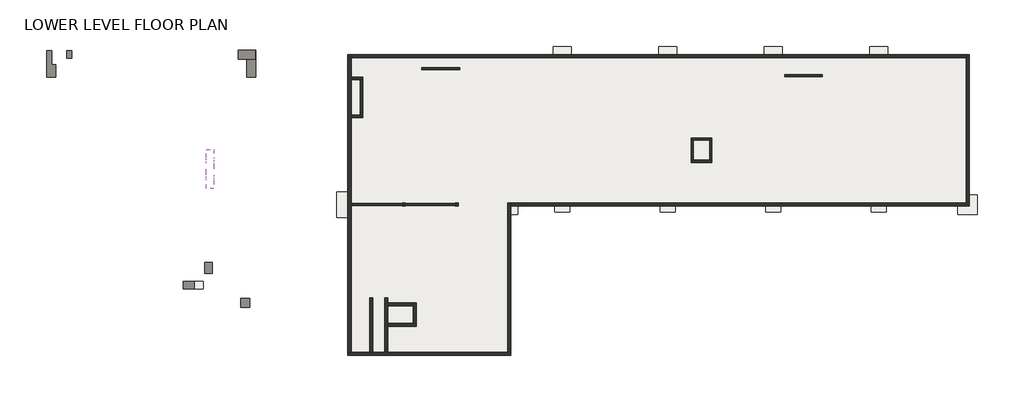
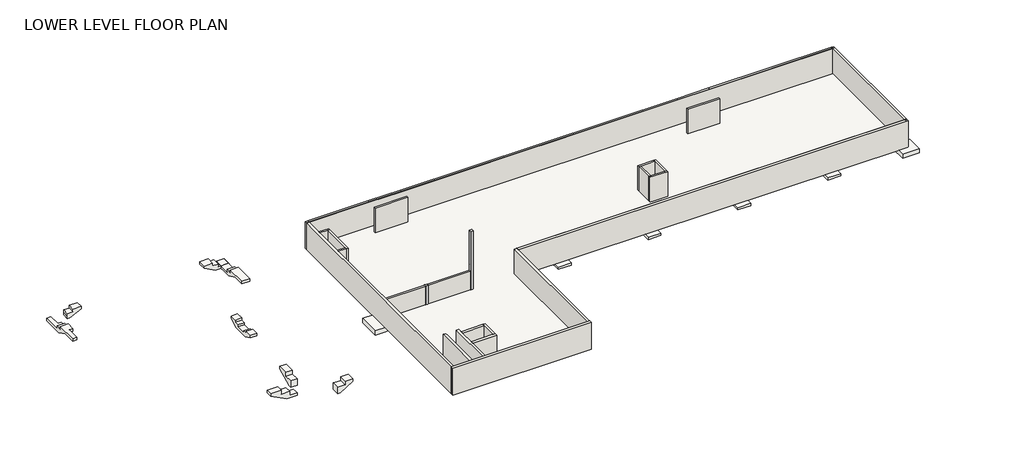
# One storey: 22 slabs, 22 walls, 2 columns.
"""IFC4 building model written with IfcOpenShell, lengths in millimetres."""

import ifcopenshell
import ifcopenshell.guid

model = None  # the IFC model being written
_history = None  # IfcOwnerHistory: only IFC2X3 demands one
_inside = {}  # id of a spatial element -> (the spatial element, [elements in it])
_under = {}  # id of a project, library or spatial element -> (it, [spatial elements below it])
_declared = {}  # id of a project -> (the project, [libraries it declares])
_typed = {}  # id of a type object -> (the type object, [elements of that type])
_made_of = {}  # id of a material, layer set ... -> (it, [elements and type objects made of it])


def new_model(schema):
    """Start an empty IFC model of exactly this schema.

    Asked for "IFC4X3", IfcOpenShell would pick the latest addendum, in which some entities
    have other attributes; the version numbers below select the first issue.
    IFC2X3 requires an IfcOwnerHistory on every rooted entity: one is made here for all.
    """
    global model, _history
    if schema == "IFC4X3":
        model = ifcopenshell.file(schema_version=(4, 3, 0, 0))
    else:
        model = ifcopenshell.file(schema=schema)
    _inside.clear()
    _under.clear()
    _declared.clear()
    _typed.clear()
    _made_of.clear()
    _history = None
    if model.schema == "IFC2X3":
        org = make("IfcOrganization", Name="unknown")
        user = make(
            "IfcPersonAndOrganization",
            ThePerson=make("IfcPerson", FamilyName="unknown"),
            TheOrganization=org,
        )
        app = make(
            "IfcApplication",
            ApplicationDeveloper=org,
            Version="unknown",
            ApplicationFullName="unknown",
            ApplicationIdentifier="unknown",
        )
        _history = make(
            "IfcOwnerHistory",
            OwningUser=user,
            OwningApplication=app,
            ChangeAction="ADDED",
            CreationDate=0,
        )
    return model


def make(cls, **values):
    """One entity of the class cls with the attributes given. An attribute that is None is left unset."""
    return model.create_entity(
        cls, **{name: value for name, value in values.items() if value is not None}
    )


def rooted(cls, **values):
    """An entity with a GlobalId (a new one), such as an element, a storey or a relation."""
    return make(cls, GlobalId=ifcopenshell.guid.new(), OwnerHistory=_history, **values)


def si_unit(unit_type, name, prefix=None):
    """IfcSIUnit, for example si_unit("LENGTHUNIT", "METRE", prefix="MILLI")."""
    return make("IfcSIUnit", UnitType=unit_type, Prefix=prefix, Name=name)


def assignment(units):
    """IfcUnitAssignment: the units of a project."""
    return None if units is None else make("IfcUnitAssignment", Units=units)


def point(xyz):
    """IfcCartesianPoint."""
    return None if xyz is None else make("IfcCartesianPoint", Coordinates=xyz)


def direction(xyz):
    """IfcDirection."""
    return None if xyz is None else make("IfcDirection", DirectionRatios=xyz)


def frame(location, z_axis=None, x_axis=None):
    """IfcAxis2Placement3D, a coordinate frame: its origin and axes. An axis left out is left unset."""
    return make(
        "IfcAxis2Placement3D",
        Location=point(location),
        Axis=direction(z_axis),
        RefDirection=direction(x_axis),
    )


def origin():
    """The frame at (0, 0, 0) with its axes left unset."""
    return frame((0.0, 0.0, 0.0))


def place(relative_to, where):
    """IfcLocalPlacement: puts the frame where relative to a parent placement (None: the world)."""
    return make(
        "IfcLocalPlacement", PlacementRelTo=relative_to, RelativePlacement=where
    )


def context(
    kind, dimensions, precision=None, world=None, true_north=None, identifier=None
):
    """IfcGeometricRepresentationContext, for example the 3D "Model" context."""
    return make(
        "IfcGeometricRepresentationContext",
        ContextIdentifier=identifier,
        ContextType=kind,
        CoordinateSpaceDimension=dimensions,
        Precision=precision,
        WorldCoordinateSystem=world,
        TrueNorth=true_north,
    )


def project(units=None, contexts=None):
    """IfcProject with its units and contexts."""
    return rooted(
        "IfcProject",
        Name="project",
        RepresentationContexts=contexts,
        UnitsInContext=assignment(units),
    )


def spatial(cls, under=None, at=None, **own):
    """A site, building, storey or space (cls), placed at a placement, below another one or the project."""
    s = rooted(cls, ObjectPlacement=at, **own)
    if under is not None:
        _under.setdefault(under.id(), (under, []))[1].append(s)
    return s


def polyline(points):
    """IfcPolyline through the points."""
    return make("IfcPolyline", Points=[point(p) for p in points])


def outline(outer, holes=None, kind="AREA"):
    """IfcArbitraryClosedProfileDef: a profile drawn as a closed curve; with holes, ...WithVoids."""
    if holes is None:
        return make("IfcArbitraryClosedProfileDef", ProfileType=kind, OuterCurve=outer)
    return make(
        "IfcArbitraryProfileDefWithVoids",
        ProfileType=kind,
        OuterCurve=outer,
        InnerCurves=holes,
    )


def extrude(swept, where, along, depth):
    """IfcExtrudedAreaSolid: the profile swept, set in the frame where, extruded along a direction by depth."""
    return make(
        "IfcExtrudedAreaSolid",
        SweptArea=swept,
        Position=where,
        ExtrudedDirection=direction(along),
        Depth=depth,
    )


def faces_of(points, faces, orient=None, outer=None):
    """IfcFace entities. A face is a list of loops; a loop is a list of indices into points, from 0.

    orient and outer hold one flag for each loop. By default every Orientation is true, the
    first loop of a face is its IfcFaceOuterBound and the others are IfcFaceBound.
    """
    made = []
    for i, loops in enumerate(faces):
        bounds = []
        for j, loop in enumerate(loops):
            is_outer = j == 0 if outer is None else outer[i][j]
            bounds.append(
                make(
                    "IfcFaceOuterBound" if is_outer else "IfcFaceBound",
                    Bound=make("IfcPolyLoop", Polygon=[points[k] for k in loop]),
                    Orientation=True if orient is None else orient[i][j],
                )
            )
        made.append(make("IfcFace", Bounds=bounds))
    return made


def faceted_brep(points, faces, orient=None, outer=None, voids=None):
    """IfcFacetedBrep: a solid bounded by flat faces; with voids (closed shells), ...WithVoids."""
    shared = [point(p) for p in points]
    hull = make("IfcClosedShell", CfsFaces=faces_of(shared, faces, orient, outer))
    if voids is None:
        return make("IfcFacetedBrep", Outer=hull)
    return make(
        "IfcFacetedBrepWithVoids",
        Outer=hull,
        Voids=[
            make(cls, CfsFaces=faces_of(shared, fs, o, b)) for cls, fs, o, b in voids
        ],
    )


def shape(context_of_items, identifier, shape_type, items):
    """IfcShapeRepresentation: the items that make up one representation, for example the "Body"."""
    return make(
        "IfcShapeRepresentation",
        ContextOfItems=context_of_items,
        RepresentationIdentifier=identifier,
        RepresentationType=shape_type,
        Items=items,
    )


def source(mapping_origin, context_of_items, identifier, shape_type, items):
    """IfcRepresentationMap: a shape defined once, which mapped items show again and again."""
    return make(
        "IfcRepresentationMap",
        MappingOrigin=mapping_origin,
        MappedRepresentation=shape(context_of_items, identifier, shape_type, items),
    )


def transform(
    local_origin,
    x_axis=None,
    y_axis=None,
    z_axis=None,
    scale=None,
    scale2=None,
    scale3=None,
    uniform=True,
):
    """IfcCartesianTransformationOperator3D, or its non-uniform kind. x_axis, y_axis, z_axis: its Axis1, 2, 3."""
    if uniform:
        return make(
            "IfcCartesianTransformationOperator3D",
            Axis1=direction(x_axis),
            Axis2=direction(y_axis),
            LocalOrigin=point(local_origin),
            Scale=scale,
            Axis3=direction(z_axis),
        )
    return make(
        "IfcCartesianTransformationOperator3DnonUniform",
        Axis1=direction(x_axis),
        Axis2=direction(y_axis),
        LocalOrigin=point(local_origin),
        Scale=scale,
        Axis3=direction(z_axis),
        Scale2=scale2,
        Scale3=scale3,
    )


def mapped(mapping_source, mapping_target):
    """IfcMappedItem: shows the shape of a source again, moved by a transform."""
    return make(
        "IfcMappedItem", MappingSource=mapping_source, MappingTarget=mapping_target
    )


def made_of(thing, what):
    """Note that an element or type object is made of a material, layer set ...; save() writes the relation."""
    if what is not None:
        _made_of.setdefault(what.id(), (what, []))[1].append(thing)
    return thing


def element(
    cls,
    number,
    at=None,
    inside=None,
    cuts=None,
    type_object=None,
    material=None,
    context=None,
    identifier="Body",
    shape_type=None,
    held_by="IfcProductDefinitionShape",
    body=None,
    shapes=None,
    **own,
):
    """One element of the class cls, such as IfcWall. Its Tag is "e" and its number.

    at: its placement. inside: the storey or other place that contains it. cuts: it is an
    opening in that element (IfcRelVoidsElement). A single representation is given by context,
    identifier, shape_type and body (its items); several are given by shapes. held_by: the class
    of the entity that holds the representations. save() writes the other relations.
    """
    e = rooted(cls, Tag="e%d" % number, ObjectPlacement=at, **own)
    if body is not None:
        shapes = [shape(context, identifier, shape_type, body)]
    if shapes is not None:
        e.Representation = make(held_by, Representations=shapes)
    if inside is not None:
        _inside.setdefault(inside.id(), (inside, []))[1].append(e)
    if cuts is not None:
        rooted(
            "IfcRelVoidsElement", RelatingBuildingElement=cuts, RelatedOpeningElement=e
        )
    if type_object is not None:
        _typed.setdefault(type_object.id(), (type_object, []))[1].append(e)
    return made_of(e, material)


def aggregate(whole, parts):
    """IfcRelAggregates: a whole, such as a stair, and the parts it consists of."""
    return rooted("IfcRelAggregates", RelatingObject=whole, RelatedObjects=parts)


def save(model, path):
    """Write the relations noted so far, then the file.

    IfcRelAggregates (storeys below a building ...), IfcRelContainedInSpatialStructure (elements
    in a storey), IfcRelDefinesByType, IfcRelAssociatesMaterial and IfcRelDeclares: one each for
    every whole, place, type object, material and project.
    """
    for whole, parts in _under.values():
        aggregate(whole, parts)
    for where, things in _inside.values():
        rooted(
            "IfcRelContainedInSpatialStructure",
            RelatedElements=things,
            RelatingStructure=where,
        )
    for kind, things in _typed.values():
        rooted("IfcRelDefinesByType", RelatedObjects=things, RelatingType=kind)
    for what, things in _made_of.values():
        rooted("IfcRelAssociatesMaterial", RelatedObjects=things, RelatingMaterial=what)
    for by, libraries in _declared.values():
        rooted("IfcRelDeclares", RelatingContext=by, RelatedDefinitions=libraries)
    model.write(path)


def footing_rectangular_4c268a4d(model_context):
    return source(origin(), model_context, "Body", "SweptSolid", [
        extrude(outline(polyline([(1295.4, 1295.4), (1295.4, -1295.4), (-1295.4, -1295.4), (-1295.4, 1295.4), (1295.4, 1295.4)])), frame((0.0, 0.0, -609.6), z_axis=(0.0, 0.0, 1.0), x_axis=(1.0, 0.0, 0.0)), (0.0, 0.0, 1.0), 609.6),
    ])


def footing_rectangular_a4ec12e7(model_context):
    return source(origin(), model_context, "Body", "SweptSolid", [
        extrude(outline(polyline([(1828.8, 1828.8), (1828.8, -1828.8), (-1828.8, -1828.8), (-1828.8, 1828.8), (1828.8, 1828.8)])), frame((0.0, 0.0, -609.6), z_axis=(0.0, 0.0, 1.0), x_axis=(1.0, 0.0, 0.0)), (0.0, 0.0, 1.0), 609.6),
    ])


def footing_rectangular_876cc71e(model_context):
    return source(origin(), model_context, "Body", "SweptSolid", [
        extrude(outline(polyline([(990.6, 990.6), (990.6, -990.6), (-990.6, -990.6), (-990.6, 990.6), (990.6, 990.6)])), frame((0.0, 0.0, -457.2), z_axis=(0.0, 0.0, 1.0), x_axis=(1.0, 0.0, 0.0)), (0.0, 0.0, 1.0), 457.2),
    ])


def footing_rectangular_0e916acc(model_context):
    return source(origin(), model_context, "Body", "SweptSolid", [
        extrude(outline(polyline([(1295.4, 1295.4), (1295.4, -1295.4), (-1295.4, -1295.4), (-1295.4, 1295.4), (1295.4, 1295.4)])), frame((0.0, 0.0, -508.0), z_axis=(0.0, 0.0, 1.0), x_axis=(1.0, 0.0, 0.0)), (0.0, 0.0, 1.0), 508.0),
    ])


def footing_rectangular_f5_f52d0094(model_context):
    return source(origin(), model_context, "Body", "SweptSolid", [
        extrude(outline(polyline([(762.0, 762.0), (762.0, -762.0), (-762.0, -762.0), (-762.0, 762.0), (762.0, 762.0)])), frame((0.0, 0.0, -304.8), z_axis=(0.0, 0.0, 1.0), x_axis=(1.0, 0.0, 0.0)), (0.0, 0.0, 1.0), 304.8),
    ])


def footing_rectangular_f6_e8c3e57f(model_context):
    return source(origin(), model_context, "Body", "SweptSolid", [
        extrude(outline(polyline([(914.4, 914.4), (914.4, -914.4), (-914.4, -914.4), (-914.4, 914.4), (914.4, 914.4)])), frame((0.0, 0.0, -304.8), z_axis=(0.0, 0.0, 1.0), x_axis=(1.0, 0.0, 0.0)), (0.0, 0.0, 1.0), 304.8),
    ])


def foundation_step_foundation_step_6eb52276(model_context):
    return source(origin(), model_context, "Body", "Brep", [
        faceted_brep([(-65781.2850821, 11238.2505048, -1422.4), (-65781.2850821, 11238.2505048, -1752.6), (-65781.2850821, 13409.3518471, -1752.6), (-65781.2850821, 13409.3518471, -2057.4), (-65781.2850821, 10933.4505048, -2057.4), (-65781.2850821, 9612.6505048, -1397.0), (-65781.2850821, 8050.5505048, -1397.0), (-65781.2850821, 8050.5505048, -1092.2), (-65781.2850821, 10577.8505048, -1092.2), (-65781.2850821, 10577.8505048, -1422.4), (-64866.8850821, 11238.2505048, -1752.6), (-64866.8850821, 11238.2505048, -1422.4), (-64866.8850821, 10577.8505048, -1422.4), (-64866.8850821, 10577.8505048, -1092.2), (-64866.8850821, 9574.5505048, -1092.2), (-64866.8850821, 9574.5505048, -1397.0), (-64866.8850821, 9612.6505048, -1397.0), (-64866.8850821, 10933.4505048, -2057.4), (-64866.8850821, 12012.9505048, -2057.4), (-64866.8850821, 12012.9505048, -1752.6), (-65273.2850821, 12012.9505048, -1752.6), (-65273.2850821, 13409.3518471, -1752.6), (-65273.2850821, 13409.3518471, -2057.4), (-65273.2850821, 12012.9505048, -2057.4), (-65273.2850821, 9574.5505048, -1397.0), (-65273.2850821, 8050.5505048, -1397.0), (-65273.2850821, 8050.5505048, -1092.2), (-65273.2850821, 9574.5505048, -1092.2)], [[[0, 1, 2, 3, 4, 5, 6, 7, 8, 9]], [[10, 11, 12, 13, 14, 15, 16, 17, 18, 19]], [[1, 0, 11, 10]], [[2, 1, 10, 19, 20, 21]], [[3, 2, 21, 22]], [[4, 3, 22, 23, 18, 17]], [[6, 5, 16, 15, 24, 25]], [[7, 6, 25, 26]], [[8, 7, 26, 27, 14, 13]], [[9, 8, 13, 12]], [[0, 9, 12, 11]], [[5, 4, 17, 16]], [[27, 24, 15, 14]], [[24, 27, 26, 25]], [[20, 23, 22, 21]], [[23, 20, 19, 18]]]),
    ])


def foundation_step1_foundation_step_c4984ecd(model_context):
    return source(origin(), model_context, "Body", "SweptSolid", [
        extrude(outline(polyline([(-1397.0, -62011.044558), (-1092.2, -62011.044558), (-1092.2, -62976.244558), (-1422.4, -62976.244558), (-1422.4, -63636.644558), (-1752.6, -63636.644558), (-1752.6, -63634.9850821), (-2057.4, -63634.9850821), (-2057.4, -63331.844558), (-1397.0, -62011.044558)])), frame((0.0, 12612.4268471, 0.0), z_axis=(0.0, 1.0, 0.0), x_axis=(0.0, 0.0, 1.0)), (0.0, 0.0, 1.0), 762.0),
    ])


def foundation_step2_foundation_step_839b83da(model_context):
    return source(origin(), model_context, "Body", "SweptSolid", [
        extrude(outline(polyline([(-1092.2, -46445.5350821), (-1092.2, -47410.7350821), (-1397.0, -47410.7350821), (-2057.4, -46089.9350821), (-2057.4, -44565.9350821), (-1752.6, -44565.9350821), (-1752.6, -45785.1350821), (-1422.4, -45785.1350821), (-1422.4, -46445.5350821), (-1092.2, -46445.5350821)])), frame((0.0, 12628.3018471, 0.0), z_axis=(0.0, 1.0, 0.0), x_axis=(0.0, 0.0, 1.0)), (0.0, 0.0, 1.0), 914.4),
    ])


def foundation_step3_foundation_step_6bcc790d(model_context):
    return source(origin(), model_context, "Body", "SweptSolid", [
        extrude(outline(polyline([(10612.1768471, -1092.2), (10612.1768471, -1422.4), (11272.5768471, -1422.4), (11272.5768471, -1752.6), (13485.5518471, -1752.6), (13485.5518471, -2057.4), (10967.7768471, -2057.4), (9646.9768471, -1397.0), (8253.7505048, -1397.0), (8253.7505048, -1092.2), (10612.1768471, -1092.2)])), frame((-45451.7600821, 0.0, 0.0), z_axis=(1.0, 0.0, 0.0), x_axis=(0.0, 1.0, 0.0)), (0.0, 0.0, 1.0), 914.4),
    ])


def foundation_step4_foundation_step_7894882b(model_context):
    return source(origin(), model_context, "Body", "SweptSolid", [
        extrude(outline(polyline([(-1092.2, -45178.5909443), (-1574.8, -45178.5909443), (-1574.8, -46054.8909443), (-2362.2, -46054.8909443), (-2362.2, -45750.0909443), (-1397.0, -44308.7600821), (-1397.0, -44302.2909443), (-1092.2, -44302.2909443), (-1092.2, -45178.5909443)])), frame((0.0, -12551.0356529, 0.0), z_axis=(0.0, 1.0, 0.0), x_axis=(0.0, 0.0, 1.0)), (0.0, 0.0, 1.0), 914.4),
    ])


def foundation_step5_foundation_step_64dcdb90(model_context):
    return source(origin(), model_context, "Body", "SweptSolid", [
        extrude(outline(polyline([(-538.4231529, -1092.2), (299.7768471, -1092.2), (299.7768471, -1358.9), (833.1768471, -1358.9), (833.1768471, -1625.6), (2052.3768471, -1625.6), (2052.3768471, -1358.9), (2585.7768471, -1358.9), (2585.7768471, -1092.2), (3423.9768471, -1092.2), (3423.9768471, -1397.0), (2357.1768471, -1930.4), (528.3768471, -1930.4), (-538.4231529, -1397.0), (-538.4231529, -1092.2)])), frame((-49531.6350821, 0.0, 0.0), z_axis=(1.0, 0.0, 0.0), x_axis=(0.0, 1.0, 0.0)), (0.0, 0.0, 1.0), 762.0),
    ])


def foundation_step6_foundation_step_ef98733d(model_context):
    return source(origin(), model_context, "Body", "SweptSolid", [
        extrude(outline(polyline([(-9123.6231529, -2362.2), (-9123.6231529, -1574.8), (-8158.4231529, -1574.8), (-8158.4231529, -1092.2), (-6888.4231529, -1092.2), (-6888.4231529, -1397.0), (-8818.8231529, -2362.2), (-9123.6231529, -2362.2)])), frame((-49611.0100821, 0.0, 0.0), z_axis=(1.0, 0.0, 0.0), x_axis=(0.0, 1.0, 0.0)), (0.0, 0.0, 1.0), 762.0),
    ])


def foundation_step7_foundation_step_1080ab70(model_context):
    return source(origin(), model_context, "Body", "SweptSolid", [
        extrude(outline(polyline([(-1092.2, -52957.4600821), (-1397.0, -52957.4600821), (-2362.2, -51027.0600821), (-2362.2, -49814.2100821), (-2057.4, -49814.2100821), (-2057.4, -50722.2600821), (-1574.8, -50722.2600821), (-1574.8, -51687.4600821), (-1092.2, -51687.4600821), (-1092.2, -52957.4600821)])), frame((0.0, -10673.0231529, 0.0), z_axis=(0.0, 1.0, 0.0), x_axis=(0.0, 0.0, 1.0)), (0.0, 0.0, 1.0), 762.0),
    ])


model = new_model("IFC4")

# Units and contexts
model_context = context("Model", 3, world=origin())
ifc_project = project(units=[si_unit("LENGTHUNIT", "METRE", prefix="MILLI")], contexts=[model_context])

# Site, building, storey
site = spatial("IfcSite", under=ifc_project)
building = spatial("IfcBuilding", under=site)
storey = spatial("IfcBuildingStorey", under=building, Name="LOWER LEVEL FLOOR PLAN", Elevation=-3149.6)

# Columns
placement = place(None, origin())
element("IfcColumn", 1, ObjectType="Concrete-Square-Column : 12 x 12", at=placement, inside=storey, context=model_context, shape_type="Brep", body=[
    faceted_brep([(-24071.1909443, -2011.6231529, -3759.2), (-24071.1909443, -2316.4231529, -3759.2), (-24375.9909443, -2316.4231529, -3759.2), (-24375.9909443, -2011.6231529, -3759.2), (-24071.1909443, -2316.4231529, -3251.2), (-24071.1909443, -2011.6231529, -3251.2), (-24375.9909443, -2011.6231529, -3251.2), (-24375.9909443, -2316.4231529, -3251.2)], [[[0, 1, 2, 3]], [[4, 5, 6, 7]], [[1, 0, 5, 4]], [[2, 1, 4, 7]], [[3, 2, 7, 6]], [[0, 3, 6, 5]]]),
    faceted_brep([(-24071.1909443, -2011.6231529, 4191.0), (-24071.1909443, -2316.4231529, 4191.0), (-24071.1909443, -2316.4231529, -3149.6), (-24071.1909443, -2011.6231529, -3149.6), (-24071.1909443, -2011.6231529, -50.8), (-24071.1909443, -2054.4856529, -50.8), (-24071.1909443, -2054.4856529, 0.0), (-24071.1909443, -2011.6231529, 0.0), (-24375.9909443, -2316.4231529, 4191.0), (-24375.9909443, -2316.4231529, -3149.6), (-24375.9909443, -2011.6231529, 4191.0), (-24375.9909443, -2011.6231529, 0.0), (-24375.9909443, -2054.4856529, 0.0), (-24375.9909443, -2054.4856529, -50.8), (-24375.9909443, -2011.6231529, -50.8), (-24375.9909443, -2011.6231529, -3149.6), (-24375.9909443, -2054.4856529, -3149.6), (-24375.9909443, -2273.5606529, -3149.6)], [[[0, 1, 2, 3, 4, 5, 6, 7]], [[1, 8, 9, 2]], [[8, 10, 11, 12, 13, 14, 15, 16, 17, 9]], [[10, 0, 7, 11]], [[1, 0, 10, 8]], [[13, 5, 4, 14]], [[6, 12, 11, 7]], [[5, 13, 12, 6]], [[3, 2, 9, 17, 16, 15]], [[14, 4, 3, 15]]]),
])
element("IfcColumn", 2, ObjectType="Concrete-Square-Column : 12 x 12", at=placement, inside=storey, context=model_context, shape_type="Brep", body=[
    faceted_brep([(-29405.1909443, -2011.6231529, -3759.2), (-29405.1909443, -2316.4231529, -3759.2), (-29709.9909443, -2316.4231529, -3759.2), (-29709.9909443, -2011.6231529, -3759.2), (-29405.1909443, -2316.4231529, -3251.2), (-29405.1909443, -2011.6231529, -3251.2), (-29709.9909443, -2011.6231529, -3251.2), (-29709.9909443, -2316.4231529, -3251.2)], [[[0, 1, 2, 3]], [[4, 5, 6, 7]], [[1, 0, 5, 4]], [[2, 1, 4, 7]], [[3, 2, 7, 6]], [[0, 3, 6, 5]]]),
    faceted_brep([(-29405.1909443, -2011.6231529, -812.8), (-29405.1909443, -2054.4856529, -812.8), (-29405.1909443, -2273.5606529, -812.8), (-29405.1909443, -2316.4231529, -812.8), (-29405.1909443, -2316.4231529, -3149.6), (-29405.1909443, -2273.5606529, -3149.6), (-29405.1909443, -2054.4856529, -3149.6), (-29405.1909443, -2011.6231529, -3149.6), (-29709.9909443, -2316.4231529, -812.8), (-29709.9909443, -2316.4231529, -3149.6), (-29709.9909443, -2273.5606529, -812.8), (-29709.9909443, -2054.4856529, -812.8), (-29709.9909443, -2011.6231529, -812.8), (-29709.9909443, -2011.6231529, -3149.6), (-29709.9909443, -2054.4856529, -3149.6), (-29709.9909443, -2273.5606529, -3149.6)], [[[0, 1, 2, 3, 4, 5, 6, 7]], [[3, 8, 9, 4]], [[8, 10, 11, 12, 13, 14, 15, 9]], [[12, 0, 7, 13]], [[3, 2, 1, 0, 12, 11, 10, 8]], [[7, 6, 5, 4, 9, 15, 14, 13]]]),
])

# Slabs
footing_rectangular_shape = footing_rectangular_4c268a4d(model_context)
element("IfcSlab", 3, ObjectType="Footing-Rectangular : F 8.5' x 8.5' x 24\"", at=placement, inside=storey, context=model_context, shape_type="MappedRepresentation", body=[
    mapped(footing_rectangular_shape, transform((-29557.5909443, -2164.0231529, -3759.2), x_axis=(1.0, 0.0, 0.0), y_axis=(0.0, 1.0, 0.0), z_axis=(0.0, 0.0, 1.0))),
])
footing_rectangular_2_shape = footing_rectangular_a4ec12e7(model_context)
element("IfcSlab", 4, ObjectType="Footing-Rectangular : E 12' x 12' x 24\"", at=placement, inside=storey, context=model_context, shape_type="MappedRepresentation", body=[
    mapped(footing_rectangular_2_shape, transform((-24223.5909443, -2164.0231529, -3759.2), x_axis=(1.0, 0.0, 0.0), y_axis=(0.0, 1.0, 0.0), z_axis=(0.0, 0.0, 1.0))),
])
footing_rectangular_3_shape = footing_rectangular_876cc71e(model_context)
element("IfcSlab", 5, ObjectType="Footing-Rectangular : D 6.5' x 6.5' x 18\"", at=placement, inside=storey, context=model_context, shape_type="MappedRepresentation", body=[
    mapped(footing_rectangular_3_shape, transform((27440.0090557, -2164.0231529, -3403.6), x_axis=(1.0, 0.0, 0.0), y_axis=(0.0, 1.0, 0.0), z_axis=(0.0, 0.0, 1.0))),
])
element("IfcSlab", 6, ObjectType="Footing-Rectangular : G 6.5' x 6.5' x 18\"", at=placement, inside=storey, context=model_context, shape_type="MappedRepresentation", body=[
    mapped(footing_rectangular_3_shape, transform((-19041.9909443, -2164.0231529, -3403.6), x_axis=(1.0, 0.0, 0.0), y_axis=(0.0, 1.0, 0.0), z_axis=(0.0, 0.0, 1.0))),
])
footing_rectangular_4_shape = footing_rectangular_0e916acc(model_context)
element("IfcSlab", 7, ObjectType="Footing-Rectangular : H 8.5' x 8.5' x 20\"", at=placement, inside=storey, context=model_context, shape_type="MappedRepresentation", body=[
    mapped(footing_rectangular_4_shape, transform((-35043.9909443, -2164.0231529, -3403.6), x_axis=(1.0, 0.0, 0.0), y_axis=(0.0, 1.0, 0.0), z_axis=(0.0, 0.0, 1.0))),
])
footing_rectangular_f5_shape = footing_rectangular_f5_f52d0094(model_context)
element("IfcSlab", 8, ObjectType="Footing-Rectangular : F5", at=placement, inside=storey, context=model_context, shape_type="MappedRepresentation", body=[
    mapped(footing_rectangular_f5_shape, transform((-13555.5909443, -2164.0231529, -3403.6), x_axis=(1.0, 0.0, 0.0), y_axis=(0.0, 1.0, 0.0), z_axis=(0.0, 0.0, 1.0))),
])
element("IfcSlab", 9, ObjectType="Footing-Rectangular : F5", at=placement, inside=storey, context=model_context, shape_type="MappedRepresentation", body=[
    mapped(footing_rectangular_f5_shape, transform((-2887.5909443, -2164.0231529, -3403.6), x_axis=(1.0, 0.0, 0.0), y_axis=(0.0, 1.0, 0.0), z_axis=(0.0, 0.0, 1.0))),
])
element("IfcSlab", 10, ObjectType="Footing-Rectangular : F5", at=placement, inside=storey, context=model_context, shape_type="MappedRepresentation", body=[
    mapped(footing_rectangular_f5_shape, transform((7780.4090557, -2164.0231529, -3403.6), x_axis=(1.0, 0.0, 0.0), y_axis=(0.0, 1.0, 0.0), z_axis=(0.0, 0.0, 1.0))),
])
element("IfcSlab", 11, ObjectType="Footing-Rectangular : F5", at=placement, inside=storey, context=model_context, shape_type="MappedRepresentation", body=[
    mapped(footing_rectangular_f5_shape, transform((18448.4090557, -2164.0231529, -3403.6), x_axis=(1.0, 0.0, 0.0), y_axis=(0.0, 1.0, 0.0), z_axis=(0.0, 0.0, 1.0))),
])
footing_rectangular_f6_shape = footing_rectangular_f6_e8c3e57f(model_context)
element("IfcSlab", 12, ObjectType="Footing-Rectangular : F6", at=placement, inside=storey, context=model_context, shape_type="MappedRepresentation", body=[
    mapped(footing_rectangular_f6_shape, transform((-13555.5909443, 12923.5768471, -3403.6), x_axis=(1.0, 0.0, 0.0), y_axis=(0.0, 1.0, 0.0), z_axis=(0.0, 0.0, 1.0))),
])
element("IfcSlab", 13, ObjectType="Footing-Rectangular : F6", at=placement, inside=storey, context=model_context, shape_type="MappedRepresentation", body=[
    mapped(footing_rectangular_f6_shape, transform((-2887.5909443, 12923.5768471, -3403.6), x_axis=(1.0, 0.0, 0.0), y_axis=(0.0, 1.0, 0.0), z_axis=(0.0, 0.0, 1.0))),
])
element("IfcSlab", 14, ObjectType="Footing-Rectangular : F6", at=placement, inside=storey, context=model_context, shape_type="MappedRepresentation", body=[
    mapped(footing_rectangular_f6_shape, transform((7780.4090557, 12923.5768471, -3403.6), x_axis=(1.0, 0.0, 0.0), y_axis=(0.0, 1.0, 0.0), z_axis=(0.0, 0.0, 1.0))),
])
element("IfcSlab", 15, ObjectType="Footing-Rectangular : F6", at=placement, inside=storey, context=model_context, shape_type="MappedRepresentation", body=[
    mapped(footing_rectangular_f6_shape, transform((18448.4090557, 12923.5768471, -3403.6), x_axis=(1.0, 0.0, 0.0), y_axis=(0.0, 1.0, 0.0), z_axis=(0.0, 0.0, 1.0))),
])
foundation_step_foundation_step_shape = foundation_step_foundation_step_6eb52276(model_context)
element("IfcSlab", 16, ObjectType="Foundation Step : Foundation Step", at=placement, inside=storey, context=model_context, shape_type="MappedRepresentation", body=[
    mapped(foundation_step_foundation_step_shape, transform((114.3, 0.0, 0.0), x_axis=(1.0, 0.0, 0.0), y_axis=(0.0, 1.0, 0.0), z_axis=(0.0, 0.0, 1.0))),
])
foundation_step1_foundation_step_shape = foundation_step1_foundation_step_c4984ecd(model_context)
element("IfcSlab", 17, ObjectType="Foundation Step1 : Foundation Step", at=placement, inside=storey, context=model_context, shape_type="MappedRepresentation", body=[
    mapped(foundation_step1_foundation_step_shape, transform((0.0, 35.5236578, 0.0), x_axis=(1.0, 0.0, 0.0), y_axis=(0.0, 1.0, 0.0), z_axis=(0.0, 0.0, 1.0))),
])
foundation_step2_foundation_step_shape = foundation_step2_foundation_step_839b83da(model_context)
element("IfcSlab", 18, ObjectType="Foundation Step2 : Foundation Step", at=placement, inside=storey, context=model_context, shape_type="MappedRepresentation", body=[
    mapped(foundation_step2_foundation_step_shape, transform((0.0, -56.5513422, 0.0), x_axis=(1.0, 0.0, 0.0), y_axis=(0.0, 1.0, 0.0), z_axis=(0.0, 0.0, 1.0))),
])
foundation_step3_foundation_step_shape = foundation_step3_foundation_step_6bcc790d(model_context)
element("IfcSlab", 19, ObjectType="Foundation Step3 : Foundation Step", at=placement, inside=storey, context=model_context, shape_type="MappedRepresentation", body=[
    mapped(foundation_step3_foundation_step_shape, transform((0.0, 0.0, 0.0), x_axis=(1.0, 0.0, 0.0), y_axis=(0.0, 1.0, 0.0), z_axis=(0.0, 0.0, 1.0))),
])
foundation_step4_foundation_step_shape = foundation_step4_foundation_step_7894882b(model_context)
element("IfcSlab", 20, ObjectType="Foundation Step4 : Foundation Step", at=placement, inside=storey, context=model_context, shape_type="MappedRepresentation", body=[
    mapped(foundation_step4_foundation_step_shape, transform((0.0, 0.0, 0.0), x_axis=(1.0, 0.0, 0.0), y_axis=(0.0, 1.0, 0.0), z_axis=(0.0, 0.0, 1.0))),
])
foundation_step5_foundation_step_shape = foundation_step5_foundation_step_64dcdb90(model_context)
element("IfcSlab", 21, ObjectType="Foundation Step5 : Foundation Step", at=placement, inside=storey, context=model_context, shape_type="MappedRepresentation", body=[
    mapped(foundation_step5_foundation_step_shape, transform((15.875, 0.0, 0.0), x_axis=(1.0, 0.0, 0.0), y_axis=(0.0, 1.0, 0.0), z_axis=(0.0, 0.0, 1.0))),
])
foundation_step6_foundation_step_shape = foundation_step6_foundation_step_ef98733d(model_context)
element("IfcSlab", 22, ObjectType="Foundation Step6 : Foundation Step", at=placement, inside=storey, context=model_context, shape_type="MappedRepresentation", body=[
    mapped(foundation_step6_foundation_step_shape, transform((-73.025, 0.0, 0.0), x_axis=(1.0, 0.0, 0.0), y_axis=(0.0, 1.0, 0.0), z_axis=(0.0, 0.0, 1.0))),
])
foundation_step7_foundation_step_shape = foundation_step7_foundation_step_1080ab70(model_context)
element("IfcSlab", 23, ObjectType="Foundation Step7 : Foundation Step", at=placement, inside=storey, context=model_context, shape_type="MappedRepresentation", body=[
    mapped(foundation_step7_foundation_step_shape, transform((0.0, -25.4, 0.0), x_axis=(1.0, 0.0, 0.0), y_axis=(0.0, 1.0, 0.0), z_axis=(0.0, 0.0, 1.0))),
])
element("IfcSlab", 24, ObjectType="SOG - 4\"", at=placement, inside=storey, context=model_context, shape_type="SweptSolid", body=[
    extrude(outline(polyline([(-34891.5909443, 12694.9768471), (27287.6090557, 12694.9768471), (27287.6090557, -2011.6231529), (-19041.9909443, -2011.6231529), (-19041.9909443, -17099.2231529), (-34891.5909443, -17099.2231529), (-34891.5909443, 12694.9768471)])), frame((0.0, 0.0, -3251.2), z_axis=(0.0, 0.0, 1.0), x_axis=(1.0, 0.0, 0.0)), (0.0, 0.0, 1.0), 101.6),
])

# Walls
element("IfcWall", 25, ObjectType="12\" CMU WALL", at=placement, inside=storey, context=model_context, shape_type="Brep", body=[
    faceted_brep([(-31170.4909443, -14473.4981529, -3403.6), (-28297.1159443, -14473.4981529, -3403.6), (-28297.1159443, -14473.4981529, -50.8), (-31170.4909443, -14473.4981529, -50.8), (-31170.4909443, -14178.2231529, -3403.6), (-31170.4909443, -14178.2231529, -50.8), (-28592.3909443, -14178.2231529, -50.8), (-28297.1159443, -14178.2231529, -50.8), (-28297.1159443, -14178.2231529, -3403.6), (-28592.3909443, -14178.2231529, -3403.6)], [[[0, 1, 2, 3]], [[4, 5, 6, 7, 8, 9]], [[1, 0, 4, 9, 8]], [[2, 1, 8, 7]], [[3, 2, 7, 6, 5]], [[0, 3, 5, 4]]]),
])
element("IfcWall", 26, ObjectType="12\" CMU WALL", at=placement, inside=storey, context=model_context, shape_type="Brep", body=[
    faceted_brep([(-28297.1159443, -14178.2231529, -3403.6), (-28297.1159443, -12104.9481529, -3403.6), (-28297.1159443, -12104.9481529, -50.8), (-28297.1159443, -14178.2231529, -50.8), (-28592.3909443, -14178.2231529, -3403.6), (-28592.3909443, -14178.2231529, -50.8), (-28592.3909443, -12400.2231529, -50.8), (-28592.3909443, -12104.9481529, -50.8), (-28592.3909443, -12104.9481529, -3403.6), (-28592.3909443, -12400.2231529, -3403.6)], [[[0, 1, 2, 3]], [[4, 5, 6, 7, 8, 9]], [[1, 0, 4, 9, 8]], [[0, 3, 5, 4]], [[2, 1, 8, 7]], [[3, 2, 7, 6, 5]]]),
])
element("IfcWall", 27, ObjectType="12\" CMU WALL", at=placement, inside=storey, context=model_context, shape_type="SweptSolid", body=[
    extrude(outline(polyline([(-31170.4909443, -12104.9481529), (-28592.3909443, -12104.9481529), (-28592.3909443, -12400.2231529), (-31170.4909443, -12400.2231529), (-31170.4909443, -12104.9481529)])), frame((0.0, 0.0, -3403.6), z_axis=(0.0, 0.0, 1.0), x_axis=(1.0, 0.0, 0.0)), (0.0, 0.0, 1.0), 3352.8),
])
element("IfcWall", 28, ObjectType="12\" CMU WALL", at=placement, inside=storey, context=model_context, shape_type="Brep", body=[
    faceted_brep([(-31465.7659443, -11612.8231529, -3403.6), (-31465.7659443, -17099.2231529, -3403.6), (-31465.7659443, -17099.2231529, -50.8), (-31465.7659443, -17086.5231529, -50.8), (-31465.7659443, -11917.6231529, -50.8), (-31465.7659443, -11612.8231529, -50.8), (-31170.4909443, -11612.8231529, -3403.6), (-31170.4909443, -11612.8231529, -50.8), (-31170.4909443, -12400.2231529, -50.8), (-31170.4909443, -14178.2231529, -50.8), (-31170.4909443, -17086.5231529, -50.8), (-31170.4909443, -17099.2231529, -50.8), (-31170.4909443, -17099.2231529, -3403.6)], [[[0, 1, 2, 3, 4, 5]], [[6, 7, 8, 9, 10, 11, 12]], [[1, 0, 6, 12]], [[0, 5, 7, 6]], [[3, 2, 11, 10]], [[2, 1, 12, 11]], [[5, 4, 3, 10, 9, 8, 7]]]),
])
element("IfcWall", 29, ObjectType="12\" CMU WALL", at=placement, inside=storey, context=model_context, shape_type="Brep", body=[
    faceted_brep([(-32999.2909443, -11612.8231529, -3403.6), (-32999.2909443, -17099.2231529, -3403.6), (-32999.2909443, -17099.2231529, -50.8), (-32999.2909443, -17086.5231529, -50.8), (-32999.2909443, -11612.8231529, -50.8), (-32704.0159443, -11612.8231529, -3403.6), (-32704.0159443, -11612.8231529, -50.8), (-32704.0159443, -11917.6231529, -50.8), (-32704.0159443, -17086.5231529, -50.8), (-32704.0159443, -17099.2231529, -50.8), (-32704.0159443, -17099.2231529, -3403.6)], [[[0, 1, 2, 3, 4]], [[5, 6, 7, 8, 9, 10]], [[1, 0, 5, 10]], [[0, 4, 6, 5]], [[2, 1, 10, 9]], [[3, 2, 9, 8]], [[4, 3, 8, 7, 6]]]),
])
element("IfcWall", 30, ObjectType="12\" CONCRETE WALL", at=placement, inside=storey, context=model_context, shape_type="Brep", body=[
    faceted_brep([(-35196.3909443, -17404.0231529, -3403.6), (-18737.1909443, -17404.0231529, -3403.6), (-18737.1909443, -17404.0231529, 0.0), (-35196.3909443, -17404.0231529, 0.0), (-35196.3909443, -17099.2231529, -3403.6), (-35196.3909443, -17099.2231529, -50.8), (-35196.3909443, -17099.2231529, 0.0), (-18737.1909443, -17099.2231529, 0.0), (-18737.1909443, -17099.2231529, -3403.6), (-34891.5909443, -17099.2231529, -3403.6)], [[[0, 1, 2, 3]], [[4, 5, 6, 7, 8, 9]], [[1, 0, 4, 9, 8]], [[3, 2, 7, 6]], [[2, 1, 8, 7]], [[0, 3, 6, 5, 4]]]),
])
element("IfcWall", 31, ObjectType="12\" CONCRETE WALL", at=placement, inside=storey, context=model_context, shape_type="Brep", body=[
    faceted_brep([(-18737.1909443, -17099.2231529, -3403.6), (-18737.1909443, -2316.4231529, -3403.6), (-18737.1909443, -2011.6231529, -3403.6), (-18737.1909443, -2011.6231529, -50.8), (-18737.1909443, -2054.4856529, -50.8), (-18737.1909443, -2316.4231529, -50.8), (-18737.1909443, -17099.2231529, -50.8), (-19041.9909443, -17099.2231529, -3403.6), (-19041.9909443, -17099.2231529, -50.8), (-19041.9909443, -2054.4856529, -50.8), (-19041.9909443, -2011.6231529, -50.8), (-19041.9909443, -2011.6231529, -3403.6)], [[[0, 1, 2, 3, 4, 5, 6]], [[7, 8, 9, 10, 11]], [[2, 1, 0, 7, 11]], [[0, 6, 8, 7]], [[3, 2, 11, 10]], [[6, 5, 4, 9, 8]], [[4, 3, 10, 9]]]),
])
element("IfcWall", 32, ObjectType="12\" CONCRETE WALL", at=placement, inside=storey, context=model_context, shape_type="Brep", body=[
    faceted_brep([(-18737.1909443, -2316.4231529, -3403.6), (27592.4090557, -2316.4231529, -3403.6), (27592.4090557, -2316.4231529, -50.8), (27338.4090557, -2316.4231529, -50.8), (-18737.1909443, -2316.4231529, -50.8), (-18737.1909443, -2011.6231529, -3403.6), (-18737.1909443, -2011.6231529, -50.8), (27287.6090557, -2011.6231529, -50.8), (27338.4090557, -2011.6231529, -50.8), (27592.4090557, -2011.6231529, -50.8), (27592.4090557, -2011.6231529, -3403.6), (27287.6090557, -2011.6231529, -3403.6), (-18737.1909443, -2054.4856529, -50.8), (27592.4090557, -2054.4856529, -50.8), (27338.4090557, -2054.4856529, -50.8)], [[[0, 1, 2, 3, 4]], [[5, 6, 7, 8, 9, 10, 11]], [[1, 0, 5, 11, 10]], [[0, 4, 12, 6, 5]], [[2, 1, 10, 9, 13]], [[13, 9, 8, 14]], [[4, 3, 14, 12]], [[3, 2, 13, 14]], [[8, 7, 6, 12, 14]]]),
])
element("IfcWall", 33, ObjectType="12\" CONCRETE WALL", at=placement, inside=storey, context=model_context, shape_type="Brep", body=[
    faceted_brep([(27592.4090557, -2011.6231529, -3403.6), (27592.4090557, 12999.7768471, -3403.6), (27592.4090557, 12999.7768471, -50.8), (27592.4090557, 12771.1768471, -50.8), (27592.4090557, -2011.6231529, -50.8), (27287.6090557, -2011.6231529, -3403.6), (27287.6090557, -2011.6231529, -50.8), (27287.6090557, 12771.1768471, -50.8), (27287.6090557, 12999.7768471, -50.8), (27287.6090557, 12999.7768471, -3403.6), (27338.4090557, -2011.6231529, -50.8), (27338.4090557, 12999.7768471, -50.8), (27338.4090557, 12771.1768471, -50.8)], [[[0, 1, 2, 3, 4]], [[5, 6, 7, 8, 9]], [[1, 0, 5, 9]], [[0, 4, 10, 6, 5]], [[2, 1, 9, 8, 11]], [[4, 3, 12, 10]], [[11, 8, 7, 12]], [[3, 2, 11, 12]], [[12, 7, 6, 10]]]),
])
element("IfcWall", 34, ObjectType="12\" CONCRETE WALL", at=placement, inside=storey, context=model_context, shape_type="Brep", body=[
    faceted_brep([(27287.6090557, 12999.7768471, -3403.6), (-35196.3909443, 12999.7768471, -3403.6), (-35196.3909443, 12999.7768471, -50.8), (-34891.5909443, 12999.7768471, -50.8), (-27741.4909443, 12999.7768471, -50.8), (-23893.3909443, 12999.7768471, -50.8), (8948.8090557, 12999.7768471, -50.8), (12758.8090557, 12999.7768471, -50.8), (27287.6090557, 12999.7768471, -50.8), (27287.6090557, 12694.9768471, -3403.6), (27287.6090557, 12694.9768471, -50.8), (12758.8090557, 12694.9768471, -50.8), (8948.8090557, 12694.9768471, -50.8), (-23893.3909443, 12694.9768471, -50.8), (-27741.4909443, 12694.9768471, -50.8), (-34891.5909443, 12694.9768471, -50.8), (-35196.3909443, 12694.9768471, -50.8), (-35196.3909443, 12694.9768471, -3403.6), (-34891.5909443, 12694.9768471, -3403.6), (27287.6090557, 12771.1768471, -50.8), (-35196.3909443, 12771.1768471, -50.8), (-34891.5909443, 12771.1768471, -50.8), (12758.8090557, 12771.1768471, -50.8), (-27741.4909443, 12771.1768471, -50.8), (-23893.3909443, 12771.1768471, -50.8), (8948.8090557, 12771.1768471, -50.8)], [[[0, 1, 2, 3, 4, 5, 6, 7, 8]], [[9, 10, 11, 12, 13, 14, 15, 16, 17, 18]], [[1, 0, 9, 18, 17]], [[0, 8, 19, 10, 9]], [[2, 1, 17, 16, 20]], [[20, 16, 15, 21]], [[3, 2, 20, 21]], [[22, 11, 10, 19]], [[4, 3, 21, 23]], [[23, 14, 13, 24]], [[5, 4, 23, 24]], [[24, 13, 12, 25]], [[6, 5, 24, 25]], [[8, 7, 22, 19]], [[25, 12, 11, 22]], [[7, 6, 25, 22]], [[21, 15, 14, 23]]]),
])
element("IfcWall", 35, ObjectType="12\" CONCRETE WALL", at=placement, inside=storey, context=model_context, shape_type="SweptSolid", body=[
    extrude(outline(polyline([(-35196.3909443, -17099.2231529), (-35196.3909443, 12694.9768471), (-34891.5909443, 12694.9768471), (-34891.5909443, -17099.2231529), (-35196.3909443, -17099.2231529)])), frame((0.0, 0.0, -3403.6), z_axis=(0.0, 0.0, 1.0), x_axis=(1.0, 0.0, 0.0)), (0.0, 0.0, 1.0), 3352.8),
])
element("IfcWall", 36, ObjectType="8\" SHEAR WALL", at=placement, inside=storey, context=model_context, shape_type="SweptSolid", body=[
    extrude(outline(polyline([(-34891.5909443, -2054.4856529), (-29709.9909443, -2054.4856529), (-29709.9909443, -2273.5606529), (-34891.5909443, -2273.5606529), (-34891.5909443, -2054.4856529)])), frame((0.0, 0.0, -3149.6), z_axis=(0.0, 0.0, 1.0), x_axis=(1.0, 0.0, 0.0)), (0.0, 0.0, 1.0), 2336.8),
])
element("IfcWall", 37, ObjectType="8\" SHEAR WALL", at=placement, inside=storey, context=model_context, shape_type="SweptSolid", body=[
    extrude(outline(polyline([(-29405.1909443, -2054.4856529), (-24375.9909443, -2054.4856529), (-24375.9909443, -2273.5606529), (-29405.1909443, -2273.5606529), (-29405.1909443, -2054.4856529)])), frame((0.0, 0.0, -3149.6), z_axis=(0.0, 0.0, 1.0), x_axis=(1.0, 0.0, 0.0)), (0.0, 0.0, 1.0), 2336.8),
])
element("IfcWall", 38, ObjectType="8\" SHEAR WALL", at=placement, inside=storey, context=model_context, shape_type="Brep", body=[
    faceted_brep([(-515.8659443, 2112.7018471, -3403.6), (1573.2840557, 2112.7018471, -3403.6), (1573.2840557, 2112.7018471, -50.8), (-515.8659443, 2112.7018471, -50.8), (-515.8659443, 2331.7768471, -3403.6), (-515.8659443, 2331.7768471, -50.8), (-296.7909443, 2331.7768471, -50.8), (1354.2090557, 2331.7768471, -50.8), (1573.2840557, 2331.7768471, -50.8), (1573.2840557, 2331.7768471, -3403.6), (1354.2090557, 2331.7768471, -3403.6), (-296.7909443, 2331.7768471, -3403.6)], [[[0, 1, 2, 3]], [[4, 5, 6, 7, 8, 9, 10, 11]], [[1, 0, 4, 11, 10, 9]], [[2, 1, 9, 8]], [[0, 3, 5, 4]], [[3, 2, 8, 7, 6, 5]]]),
])
element("IfcWall", 39, ObjectType="8\" SHEAR WALL", at=placement, inside=storey, context=model_context, shape_type="Brep", body=[
    faceted_brep([(1573.2840557, 2331.7768471, -3403.6), (1573.2840557, 4582.8518471, -3403.6), (1573.2840557, 4582.8518471, -50.8), (1573.2840557, 2331.7768471, -50.8), (1354.2090557, 2331.7768471, -3403.6), (1354.2090557, 2331.7768471, -50.8), (1354.2090557, 4363.7768471, -50.8), (1354.2090557, 4582.8518471, -50.8), (1354.2090557, 4582.8518471, -3403.6), (1354.2090557, 4363.7768471, -3403.6)], [[[0, 1, 2, 3]], [[4, 5, 6, 7, 8, 9]], [[1, 0, 4, 9, 8]], [[0, 3, 5, 4]], [[2, 1, 8, 7]], [[3, 2, 7, 6, 5]]]),
])
element("IfcWall", 40, ObjectType="8\" SHEAR WALL", at=placement, inside=storey, context=model_context, shape_type="Brep", body=[
    faceted_brep([(1354.2090557, 4582.8518471, -3403.6), (-515.8659443, 4582.8518471, -3403.6), (-515.8659443, 4582.8518471, -50.8), (1354.2090557, 4582.8518471, -50.8), (1354.2090557, 4363.7768471, -3403.6), (1354.2090557, 4363.7768471, -50.8), (-296.7909443, 4363.7768471, -50.8), (-515.8659443, 4363.7768471, -50.8), (-515.8659443, 4363.7768471, -3403.6), (-296.7909443, 4363.7768471, -3403.6)], [[[0, 1, 2, 3]], [[4, 5, 6, 7, 8, 9]], [[1, 0, 4, 9, 8]], [[0, 3, 5, 4]], [[2, 1, 8, 7]], [[3, 2, 7, 6, 5]]]),
])
element("IfcWall", 41, ObjectType="8\" SHEAR WALL", at=placement, inside=storey, context=model_context, shape_type="SweptSolid", body=[
    extrude(outline(polyline([(-515.8659443, 2331.7768471), (-515.8659443, 4363.7768471), (-296.7909443, 4363.7768471), (-296.7909443, 2331.7768471), (-515.8659443, 2331.7768471)])), frame((0.0, 0.0, -3403.6), z_axis=(0.0, 0.0, 1.0), x_axis=(1.0, 0.0, 0.0)), (0.0, 0.0, 1.0), 3352.8),
])
element("IfcWall", 42, ObjectType="8\" SHEAR WALL", at=placement, inside=storey, context=model_context, shape_type="SweptSolid", body=[
    extrude(outline(polyline([(12758.8090557, 10774.1018471), (8948.8090557, 10774.1018471), (8948.8090557, 10993.1768471), (12758.8090557, 10993.1768471), (12758.8090557, 10774.1018471)])), frame((0.0, 0.0, -3403.6), z_axis=(0.0, 0.0, 1.0), x_axis=(1.0, 0.0, 0.0)), (0.0, 0.0, 1.0), 3352.8),
])
element("IfcWall", 43, ObjectType="8\" SHEAR WALL", at=placement, inside=storey, context=model_context, shape_type="SweptSolid", body=[
    extrude(outline(polyline([(-23893.3909443, 11485.3018471), (-27741.4909443, 11485.3018471), (-27741.4909443, 11704.3768471), (-23893.3909443, 11704.3768471), (-23893.3909443, 11485.3018471)])), frame((0.0, 0.0, -3403.6), z_axis=(0.0, 0.0, 1.0), x_axis=(1.0, 0.0, 0.0)), (0.0, 0.0, 1.0), 3352.8),
])
element("IfcWall", 44, ObjectType="8\" SHEAR WALL", at=placement, inside=storey, context=model_context, shape_type="Brep", body=[
    faceted_brep([(-34891.5909443, 10499.7866099, -3403.6), (-33942.2659443, 10499.7866099, -3403.6), (-33723.1909443, 10499.7866099, -3403.6), (-33723.1909443, 10499.7866099, -50.8), (-33942.2659443, 10499.7866099, -50.8), (-34891.5909443, 10499.7866099, -50.8), (-34891.5909443, 10718.8616099, -3403.6), (-34891.5909443, 10718.8616099, -50.8), (-33723.1909443, 10718.8616099, -50.8), (-33723.1909443, 10718.8616099, -3403.6)], [[[0, 1, 2, 3, 4, 5]], [[6, 7, 8, 9]], [[2, 1, 0, 6, 9]], [[0, 5, 7, 6]], [[3, 2, 9, 8]], [[5, 4, 3, 8, 7]]]),
])
element("IfcWall", 45, ObjectType="8\" SHEAR WALL", at=placement, inside=storey, context=model_context, shape_type="Brep", body=[
    faceted_brep([(-33942.2659443, 10499.7866099, -3403.6), (-33942.2659443, 6873.9366099, -3403.6), (-33942.2659443, 6654.8616099, -3403.6), (-33942.2659443, 6654.8616099, -50.8), (-33942.2659443, 6873.9366099, -50.8), (-33942.2659443, 10499.7866099, -50.8), (-33723.1909443, 10499.7866099, -3403.6), (-33723.1909443, 10499.7866099, -50.8), (-33723.1909443, 6654.8616099, -50.8), (-33723.1909443, 6654.8616099, -3403.6)], [[[0, 1, 2, 3, 4, 5]], [[6, 7, 8, 9]], [[2, 1, 0, 6, 9]], [[0, 5, 7, 6]], [[3, 2, 9, 8]], [[5, 4, 3, 8, 7]]]),
])
element("IfcWall", 46, ObjectType="8\" SHEAR WALL", at=placement, inside=storey, context=model_context, shape_type="SweptSolid", body=[
    extrude(outline(polyline([(-34891.5909443, 6873.9366099), (-33942.2659443, 6873.9366099), (-33942.2659443, 6654.8616099), (-34891.5909443, 6654.8616099), (-34891.5909443, 6873.9366099)])), frame((0.0, 0.0, -3403.6), z_axis=(0.0, 0.0, 1.0), x_axis=(1.0, 0.0, 0.0)), (0.0, 0.0, 1.0), 3352.8),
])

save(model, "model.ifc")

# Revit data of these elements
# Project information
#   Workset = "Project Info"
#   Project Issue Date = "05/17/2018"
#   Project Status = "Project Status"
#   Client Name = "Owner"
#   Project Address = "4624 W Madison St.\nChicago, IL 60644"
#   Project Name = "MALCOLM X WEST SIDE LEARNING CENTER"
#   Project Number = "17047"
#   BaseFileName = "P:\\Rm114817\\Design\\Calculations\\Structural\\180129_17047 - WESTSIDE LEARNING CENTER_STR_ASelsky.rfl"
#   ExchangeFileName = "P:\\Rm114817\\Design\\Calculations\\Structural\\180129_17047 - WESTSIDE LEARNING CENTER_STR_ASelsky.exc"
# Grids (mm)
#   "15": line (-56805.56, 17373.983) -> (-56805.56, -26049.912)
#   "12.3": line (-40952.785, 17373.983) -> (-40952.785, -26049.912)
#   "A2": line (-68768.804, 8812.551) -> (-42620.008, 8812.551)
#   "B1": line (-68768.804, -1131.354) -> (-60924.883, -1131.354)
#   "D1": line (-68768.804, -10038.023) -> (-42620.008, -10038.023)
#   "7": line (-2887.591, -24519.767) -> (-2887.591, 16616.214)
#   "9": line (7780.409, -24519.767) -> (7780.409, 16616.214)
#   "11": line (18448.409, -24519.767) -> (18448.409, 16616.214)
#   "12": line (27440.009, -25311.768) -> (27440.009, 16616.214)
#   "5": line (-13555.591, -24519.767) -> (-13555.591, 16616.214)
#   "3": line (-24223.591, -26049.912) -> (-24223.591, 16616.214)
#   "1": line (-35043.991, -26049.912) -> (-35043.991, 16616.214)
#   "A": line (30280.28, 12923.577) -> (-68768.804, 12923.577)
#   "B": line (30280.28, 5379.777) -> (-68768.804, 5379.777)
#   "C": line (30280.28, -2164.023) -> (-68768.804, -2164.023)
#   "D": line (30280.28, -9707.823) -> (-68768.804, -9707.823)
#   "E": line (30280.28, -20299.623) -> (-68768.804, -20299.623)
#   "10": line (17026.009, -25311.768) -> (17026.009, 16616.214)
#   "8": line (6612.009, -25311.768) -> (6612.009, 16616.214)
#   "6": line (-3801.991, -25311.768) -> (-3801.991, 16616.214)
#   "4": line (-14215.991, -25311.768) -> (-14215.991, 16616.214)
#   "2": line (-24629.991, -26049.912) -> (-24629.991, 16616.214)
#   "EE": line (-16739.124, -20782.223) -> (-68768.804, -20782.223)
#   "1.1": line (-35424.991, 17373.983) -> (-35424.991, -25955.606)
#   "1.6": line (-30256.091, 17373.983) -> (-30256.091, -25955.606)
#   "1.8": line (-28281.241, 17373.983) -> (-28281.241, -25955.606)
#   "E1": line (-17063.817, -23804.823) -> (-70048.485, -23804.823)
#   "D4": line (-17063.817, -18064.423) -> (-70048.485, -18064.423)
#   "D3": line (-17063.817, -13555.923) -> (-70048.485, -13555.923)
#   "D2": line (-17063.817, -11917.623) -> (-70048.485, -11917.623)
#   "C1": line (-17063.817, -7345.623) -> (-70048.485, -7345.623)
#   "12.2": line (-40530.391, 17373.983) -> (-40530.391, -25955.606)
#   "12.1": line (-39463.591, 17373.983) -> (-39463.591, -25955.606)
#   "A1": line (-41676.685, 12774.951) -> (-69261.085, 12774.951)
#   "16": line (-64396.985, 17373.983) -> (-64396.985, -26049.912)
#   "14": line (-48906.16, 17373.983) -> (-48906.16, -26049.912)
#   "13": line (-45248.56, 17373.983) -> (-45248.56, -26049.912)
#   "CC": line (-16739.124, -4551.623) -> (-68768.804, -4551.623)
# Type "Concrete-Square-Column : 12 x 12"
#   Assembly Code = "B10"
#   b = 1' - 0"
#   Structural Material [instance default] = Concrete, Cast-in-Place gray
# Type "Footing-Rectangular : F 8.5' x 8.5' x 24\""
#   Assembly Code = "A1010100"
#   Width = 8' - 6"
#   Length = 8' - 6"
#   Foundation Thickness = 2' - 0"
#   Structural Material [instance default] = Concrete, Cast-in-Place gray
# Type "Footing-Rectangular : E 12' x 12' x 24\""
#   Assembly Code = "A1010100"
#   Width = 12' - 0"
#   Length = 12' - 0"
#   Foundation Thickness = 2' - 0"
#   Structural Material [instance default] = Concrete, Cast-in-Place gray
# Type "Footing-Rectangular : D 6.5' x 6.5' x 18\""
#   Assembly Code = "A1010100"
#   Width = 6' - 6"
#   Length = 6' - 6"
#   Foundation Thickness = 1' - 6"
#   Structural Material [instance default] = Concrete, Cast-in-Place gray
# Type "Footing-Rectangular : G 6.5' x 6.5' x 18\""
#   Assembly Code = "A1010100"
#   Width = 6' - 6"
#   Length = 6' - 6"
#   Foundation Thickness = 1' - 6"
#   Structural Material [instance default] = Concrete, Cast-in-Place gray
# Type "Footing-Rectangular : H 8.5' x 8.5' x 20\""
#   Assembly Code = "A1010100"
#   Width = 8' - 6"
#   Length = 8' - 6"
#   Foundation Thickness = 1' - 8"
#   Structural Material [instance default] = Concrete, Cast-in-Place gray
# Type "Footing-Rectangular : F5"
#   Assembly Code = "A1010100"
#   Width = 5' - 0"
#   Length = 5' - 0"
#   Foundation Thickness = 1' - 0"
#   Structural Material [instance default] = Concrete, Cast-in-Place gray
# Type "Footing-Rectangular : F6"
#   Assembly Code = "A1010100"
#   Width = 6' - 0"
#   Length = 6' - 0"
#   Foundation Thickness = 1' - 0"
#   Structural Material [instance default] = Concrete, Cast-in-Place gray
# Type "Foundation Step : Foundation Step"
#   Structural Material = Concrete, Cast-in-Place gray
# Type "Foundation Step1 : Foundation Step"
#   Structural Material = Concrete, Cast-in-Place gray
# Type "Foundation Step2 : Foundation Step"
#   Structural Material = Concrete, Cast-in-Place gray
# Type "Foundation Step3 : Foundation Step"
#   Structural Material = Concrete, Cast-in-Place gray
# Type "Foundation Step4 : Foundation Step"
#   Structural Material = Concrete, Cast-in-Place gray
# Type "Foundation Step5 : Foundation Step"
#   Structural Material = Concrete, Cast-in-Place gray
# Type "Foundation Step6 : Foundation Step"
#   Structural Material = Concrete, Cast-in-Place gray
# Type "Foundation Step7 : Foundation Step"
#   Structural Material = Concrete, Cast-in-Place gray
# Type "SOG - 4\""
#   Assembly Code = "B1010"
#   Function = 0
#   Layers, outside or top first: 0' - 4" no material (function 1)
# Type "12\" CMU WALL"
#   Assembly Code = "B2010158"
#   Layers, outside or top first: 0' - 11 5/8" "Concrete Masonry Units" (function 1)
# Type "12\" CONCRETE WALL"
#   Assembly Code = "B2010158"
#   Layers, outside or top first: 1' - 0" "Concrete, Cast-in-Place gray" (function 1)
# Type "8\" SHEAR WALL"
#   Assembly Code = "B2010158"
#   Layers, outside or top first: 0' - 8 5/8" "Concrete Masonry Units" (function 1)
# Elements 1, 2 (IfcColumn, "Concrete-Square-Column : 12 x 12")
#   Structural Material = Concrete, Cast-in-Place gray
#   Phase Created = Existing
#   Materials on its faces: "Concrete, Cast-in-Place gray"
# Element 3 (IfcSlab, "Footing-Rectangular : F 8.5' x 8.5' x 24\"")
#   Structural Material = Concrete, Cast-in-Place gray
#   Phase Created = New Construction
#   Materials on its faces: "Concrete, Cast-in-Place gray"
# Element 4 (IfcSlab, "Footing-Rectangular : E 12' x 12' x 24\"")
#   Structural Material = Concrete, Cast-in-Place gray
#   Phase Created = New Construction
#   Materials on its faces: "Concrete, Cast-in-Place gray"
# Element 5 (IfcSlab, "Footing-Rectangular : D 6.5' x 6.5' x 18\"")
#   Structural Material = Concrete, Cast-in-Place gray
#   Phase Created = New Construction
#   Materials on its faces: "Concrete, Cast-in-Place gray"
# Element 6 (IfcSlab, "Footing-Rectangular : G 6.5' x 6.5' x 18\"")
#   Structural Material = Concrete, Cast-in-Place gray
#   Phase Created = New Construction
#   Materials on its faces: "Concrete, Cast-in-Place gray"
# Element 7 (IfcSlab, "Footing-Rectangular : H 8.5' x 8.5' x 20\"")
#   Structural Material = Concrete, Cast-in-Place gray
#   Phase Created = New Construction
#   Materials on its faces: "Concrete, Cast-in-Place gray"
# Elements 8, 9, 10, 11 (IfcSlab, "Footing-Rectangular : F5")
#   Structural Material = Concrete, Cast-in-Place gray
#   Phase Created = New Construction
#   Materials on its faces: "Concrete, Cast-in-Place gray"
# Elements 12, 13, 14, 15 (IfcSlab, "Footing-Rectangular : F6")
#   Structural Material = Concrete, Cast-in-Place gray
#   Phase Created = New Construction
#   Materials on its faces: "Concrete, Cast-in-Place gray"
# Element 16 (IfcSlab, "Foundation Step : Foundation Step")
#   Phase Created = New Construction
# Element 17 (IfcSlab, "Foundation Step1 : Foundation Step")
#   Phase Created = New Construction
# Element 18 (IfcSlab, "Foundation Step2 : Foundation Step")
#   Phase Created = New Construction
# Element 19 (IfcSlab, "Foundation Step3 : Foundation Step")
#   Phase Created = New Construction
# Element 20 (IfcSlab, "Foundation Step4 : Foundation Step")
#   Phase Created = New Construction
# Element 21 (IfcSlab, "Foundation Step5 : Foundation Step")
#   Phase Created = New Construction
# Element 22 (IfcSlab, "Foundation Step6 : Foundation Step")
#   Phase Created = New Construction
# Element 23 (IfcSlab, "Foundation Step7 : Foundation Step")
#   Phase Created = New Construction
# Element 24 (IfcSlab, "SOG - 4\"")
#   built-in parameter 1001955 = 1.5708 (stored number, unit not read)
#   Height Offset From Level = 0' - 0"
#   built-in parameter 1001954 = 1
#   Phase Created = Existing
# Elements 25, 26, 27 (IfcWall, "12\" CMU WALL")
#   Comments = ""
#   built-in parameter 1001111 = -0' - 10"
#   Top Offset = 0' - 0"
#   Base Offset = -0' - 10"
#   wall height = 11' - 0"
#   Phase Created = Existing
#   Base Constraint = LOWER LEVEL FLOOR PLAN
#   Top Constraint = MAIN LEVEL FLOOR PLAN
#   Materials on its faces: "Concrete Masonry Units"
# Elements 28, 29 (IfcWall, "12\" CMU WALL")
#   Comments = ""
#   built-in parameter 1001111 = -0' - 10"
#   Top Offset = 0' - 0"
#   Base Offset = -0' - 10"
#   wall height = 11' - 0"
#   Phase Created = New Construction
#   Base Constraint = LOWER LEVEL FLOOR PLAN
#   Top Constraint = MAIN LEVEL FLOOR PLAN
#   Materials on its faces: "Concrete Masonry Units"
# Element 30 (IfcWall, "12\" CONCRETE WALL")
#   Comments = ""
#   built-in parameter 1001111 = -0' - 10"
#   Top Offset = 0' - 0"
#   Base Offset = -0' - 10"
#   wall height = 11' - 2"
#   Phase Created = Existing
#   Base Constraint = LOWER LEVEL FLOOR PLAN
#   Top Constraint = MAIN LEVEL FLOOR PLAN
#   Materials on its faces: "Concrete, Cast-in-Place gray"
# Elements 31, 32, 33 (IfcWall, "12\" CONCRETE WALL")
#   Comments = ""
#   built-in parameter 1001111 = -0' - 10"
#   Top Offset = 0' - 0"
#   Base Offset = -0' - 10"
#   wall height = 11' - 0"
#   Phase Created = New Construction
#   Base Constraint = LOWER LEVEL FLOOR PLAN
#   Top Constraint = MAIN LEVEL FLOOR PLAN
#   Materials on its faces: "Concrete, Cast-in-Place gray"
# Elements 34, 35 (IfcWall, "12\" CONCRETE WALL")
#   Comments = ""
#   built-in parameter 1001111 = -0' - 10"
#   Top Offset = 0' - 0"
#   Base Offset = -0' - 10"
#   wall height = 11' - 0"
#   Phase Created = Existing
#   Base Constraint = LOWER LEVEL FLOOR PLAN
#   Top Constraint = MAIN LEVEL FLOOR PLAN
#   Materials on its faces: "Concrete, Cast-in-Place gray"
# Elements 36, 37 (IfcWall, "8\" SHEAR WALL")
#   Comments = ""
#   Top Offset = -2' - 8"
#   Base Offset = 0' - 0"
#   wall height = 7' - 8"
#   Phase Created = Existing
#   Base Constraint = LOWER LEVEL FLOOR PLAN
#   Top Constraint = MAIN LEVEL FLOOR PLAN
#   Materials on its faces: "Concrete Masonry Units"
# Elements 38, 39, 40, 41, 42, 43, 44, 45, 46 (IfcWall, "8\" SHEAR WALL")
#   Comments = ""
#   built-in parameter 1001111 = -0' - 10"
#   Top Offset = 0' - 0"
#   Base Offset = -0' - 10"
#   wall height = 11' - 0"
#   Phase Created = New Construction
#   Base Constraint = LOWER LEVEL FLOOR PLAN
#   Top Constraint = MAIN LEVEL FLOOR PLAN
#   Materials on its faces: "Concrete Masonry Units"
# Materials
#   "Concrete, Cast-in-Place gray": class "Concrete", colour RGB 192 192 192, transparency 0, Description = "Cast-in-place concrete", Cost = 0
#   "Concrete Masonry Units": class "Masonry", colour RGB 227 227 227, transparency 0, Description = "Concrete masonry units", Cost = 0
